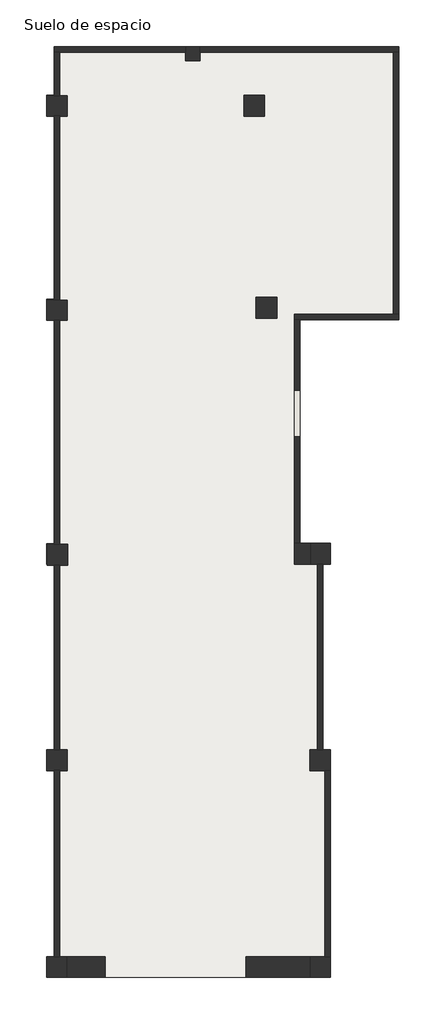
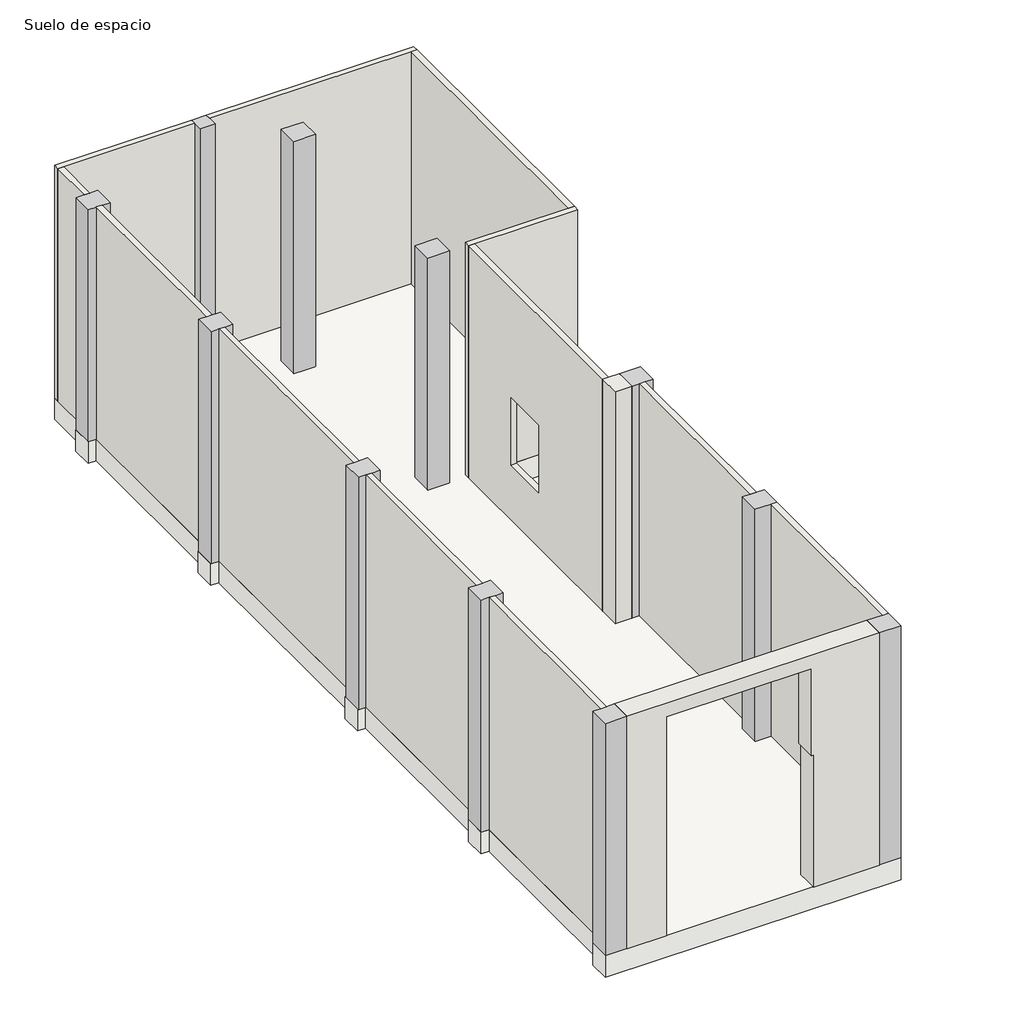
# One storey: 14 walls, 11 columns, 1 slab.
"""IFC4 building model written with IfcOpenShell, lengths in millimetres."""

import ifcopenshell
import ifcopenshell.guid

model = None  # the IFC model being written
_history = None  # IfcOwnerHistory: only IFC2X3 demands one
_inside = {}  # id of a spatial element -> (the spatial element, [elements in it])
_under = {}  # id of a project, library or spatial element -> (it, [spatial elements below it])
_declared = {}  # id of a project -> (the project, [libraries it declares])
_typed = {}  # id of a type object -> (the type object, [elements of that type])
_made_of = {}  # id of a material, layer set ... -> (it, [elements and type objects made of it])


def new_model(schema):
    """Start an empty IFC model of exactly this schema.

    Asked for "IFC4X3", IfcOpenShell would pick the latest addendum, in which some entities
    have other attributes; the version numbers below select the first issue.
    IFC2X3 requires an IfcOwnerHistory on every rooted entity: one is made here for all.
    """
    global model, _history
    if schema == "IFC4X3":
        model = ifcopenshell.file(schema_version=(4, 3, 0, 0))
    else:
        model = ifcopenshell.file(schema=schema)
    _inside.clear()
    _under.clear()
    _declared.clear()
    _typed.clear()
    _made_of.clear()
    _history = None
    if model.schema == "IFC2X3":
        org = make("IfcOrganization", Name="unknown")
        user = make(
            "IfcPersonAndOrganization",
            ThePerson=make("IfcPerson", FamilyName="unknown"),
            TheOrganization=org,
        )
        app = make(
            "IfcApplication",
            ApplicationDeveloper=org,
            Version="unknown",
            ApplicationFullName="unknown",
            ApplicationIdentifier="unknown",
        )
        _history = make(
            "IfcOwnerHistory",
            OwningUser=user,
            OwningApplication=app,
            ChangeAction="ADDED",
            CreationDate=0,
        )
    return model


def make(cls, **values):
    """One entity of the class cls with the attributes given. An attribute that is None is left unset."""
    return model.create_entity(
        cls, **{name: value for name, value in values.items() if value is not None}
    )


def rooted(cls, **values):
    """An entity with a GlobalId (a new one), such as an element, a storey or a relation."""
    return make(cls, GlobalId=ifcopenshell.guid.new(), OwnerHistory=_history, **values)


def si_unit(unit_type, name, prefix=None):
    """IfcSIUnit, for example si_unit("LENGTHUNIT", "METRE", prefix="MILLI")."""
    return make("IfcSIUnit", UnitType=unit_type, Prefix=prefix, Name=name)


def assignment(units):
    """IfcUnitAssignment: the units of a project."""
    return None if units is None else make("IfcUnitAssignment", Units=units)


def point(xyz):
    """IfcCartesianPoint."""
    return None if xyz is None else make("IfcCartesianPoint", Coordinates=xyz)


def direction(xyz):
    """IfcDirection."""
    return None if xyz is None else make("IfcDirection", DirectionRatios=xyz)


def frame(location, z_axis=None, x_axis=None):
    """IfcAxis2Placement3D, a coordinate frame: its origin and axes. An axis left out is left unset."""
    return make(
        "IfcAxis2Placement3D",
        Location=point(location),
        Axis=direction(z_axis),
        RefDirection=direction(x_axis),
    )


def origin():
    """The frame at (0, 0, 0) with its axes left unset."""
    return frame((0.0, 0.0, 0.0))


def origin_with_axes():
    """The frame at (0, 0, 0) with the z axis (0, 0, 1) and the x axis (1, 0, 0) written out."""
    return frame((0.0, 0.0, 0.0), z_axis=(0.0, 0.0, 1.0), x_axis=(1.0, 0.0, 0.0))


def place(relative_to, where):
    """IfcLocalPlacement: puts the frame where relative to a parent placement (None: the world)."""
    return make(
        "IfcLocalPlacement", PlacementRelTo=relative_to, RelativePlacement=where
    )


def context(
    kind, dimensions, precision=None, world=None, true_north=None, identifier=None
):
    """IfcGeometricRepresentationContext, for example the 3D "Model" context."""
    return make(
        "IfcGeometricRepresentationContext",
        ContextIdentifier=identifier,
        ContextType=kind,
        CoordinateSpaceDimension=dimensions,
        Precision=precision,
        WorldCoordinateSystem=world,
        TrueNorth=true_north,
    )


def project(units=None, contexts=None):
    """IfcProject with its units and contexts."""
    return rooted(
        "IfcProject",
        Name="project",
        RepresentationContexts=contexts,
        UnitsInContext=assignment(units),
    )


def spatial(cls, under=None, at=None, **own):
    """A site, building, storey or space (cls), placed at a placement, below another one or the project."""
    s = rooted(cls, ObjectPlacement=at, **own)
    if under is not None:
        _under.setdefault(under.id(), (under, []))[1].append(s)
    return s


def polyline(points):
    """IfcPolyline through the points."""
    return make("IfcPolyline", Points=[point(p) for p in points])


def outline(outer, holes=None, kind="AREA"):
    """IfcArbitraryClosedProfileDef: a profile drawn as a closed curve; with holes, ...WithVoids."""
    if holes is None:
        return make("IfcArbitraryClosedProfileDef", ProfileType=kind, OuterCurve=outer)
    return make(
        "IfcArbitraryProfileDefWithVoids",
        ProfileType=kind,
        OuterCurve=outer,
        InnerCurves=holes,
    )


def extrude(swept, where, along, depth):
    """IfcExtrudedAreaSolid: the profile swept, set in the frame where, extruded along a direction by depth."""
    return make(
        "IfcExtrudedAreaSolid",
        SweptArea=swept,
        Position=where,
        ExtrudedDirection=direction(along),
        Depth=depth,
    )


def faces_of(points, faces, orient=None, outer=None):
    """IfcFace entities. A face is a list of loops; a loop is a list of indices into points, from 0.

    orient and outer hold one flag for each loop. By default every Orientation is true, the
    first loop of a face is its IfcFaceOuterBound and the others are IfcFaceBound.
    """
    made = []
    for i, loops in enumerate(faces):
        bounds = []
        for j, loop in enumerate(loops):
            is_outer = j == 0 if outer is None else outer[i][j]
            bounds.append(
                make(
                    "IfcFaceOuterBound" if is_outer else "IfcFaceBound",
                    Bound=make("IfcPolyLoop", Polygon=[points[k] for k in loop]),
                    Orientation=True if orient is None else orient[i][j],
                )
            )
        made.append(make("IfcFace", Bounds=bounds))
    return made


def faceted_brep(points, faces, orient=None, outer=None, voids=None):
    """IfcFacetedBrep: a solid bounded by flat faces; with voids (closed shells), ...WithVoids."""
    shared = [point(p) for p in points]
    hull = make("IfcClosedShell", CfsFaces=faces_of(shared, faces, orient, outer))
    if voids is None:
        return make("IfcFacetedBrep", Outer=hull)
    return make(
        "IfcFacetedBrepWithVoids",
        Outer=hull,
        Voids=[
            make(cls, CfsFaces=faces_of(shared, fs, o, b)) for cls, fs, o, b in voids
        ],
    )


def shape(context_of_items, identifier, shape_type, items):
    """IfcShapeRepresentation: the items that make up one representation, for example the "Body"."""
    return make(
        "IfcShapeRepresentation",
        ContextOfItems=context_of_items,
        RepresentationIdentifier=identifier,
        RepresentationType=shape_type,
        Items=items,
    )


def source(mapping_origin, context_of_items, identifier, shape_type, items):
    """IfcRepresentationMap: a shape defined once, which mapped items show again and again."""
    return make(
        "IfcRepresentationMap",
        MappingOrigin=mapping_origin,
        MappedRepresentation=shape(context_of_items, identifier, shape_type, items),
    )


def transform(
    local_origin,
    x_axis=None,
    y_axis=None,
    z_axis=None,
    scale=None,
    scale2=None,
    scale3=None,
    uniform=True,
):
    """IfcCartesianTransformationOperator3D, or its non-uniform kind. x_axis, y_axis, z_axis: its Axis1, 2, 3."""
    if uniform:
        return make(
            "IfcCartesianTransformationOperator3D",
            Axis1=direction(x_axis),
            Axis2=direction(y_axis),
            LocalOrigin=point(local_origin),
            Scale=scale,
            Axis3=direction(z_axis),
        )
    return make(
        "IfcCartesianTransformationOperator3DnonUniform",
        Axis1=direction(x_axis),
        Axis2=direction(y_axis),
        LocalOrigin=point(local_origin),
        Scale=scale,
        Axis3=direction(z_axis),
        Scale2=scale2,
        Scale3=scale3,
    )


def mapped(mapping_source, mapping_target):
    """IfcMappedItem: shows the shape of a source again, moved by a transform."""
    return make(
        "IfcMappedItem", MappingSource=mapping_source, MappingTarget=mapping_target
    )


def made_of(thing, what):
    """Note that an element or type object is made of a material, layer set ...; save() writes the relation."""
    if what is not None:
        _made_of.setdefault(what.id(), (what, []))[1].append(thing)
    return thing


def element(
    cls,
    number,
    at=None,
    inside=None,
    cuts=None,
    type_object=None,
    material=None,
    context=None,
    identifier="Body",
    shape_type=None,
    held_by="IfcProductDefinitionShape",
    body=None,
    shapes=None,
    **own,
):
    """One element of the class cls, such as IfcWall. Its Tag is "e" and its number.

    at: its placement. inside: the storey or other place that contains it. cuts: it is an
    opening in that element (IfcRelVoidsElement). A single representation is given by context,
    identifier, shape_type and body (its items); several are given by shapes. held_by: the class
    of the entity that holds the representations. save() writes the other relations.
    """
    e = rooted(cls, Tag="e%d" % number, ObjectPlacement=at, **own)
    if body is not None:
        shapes = [shape(context, identifier, shape_type, body)]
    if shapes is not None:
        e.Representation = make(held_by, Representations=shapes)
    if inside is not None:
        _inside.setdefault(inside.id(), (inside, []))[1].append(e)
    if cuts is not None:
        rooted(
            "IfcRelVoidsElement", RelatingBuildingElement=cuts, RelatedOpeningElement=e
        )
    if type_object is not None:
        _typed.setdefault(type_object.id(), (type_object, []))[1].append(e)
    return made_of(e, material)


def aggregate(whole, parts):
    """IfcRelAggregates: a whole, such as a stair, and the parts it consists of."""
    return rooted("IfcRelAggregates", RelatingObject=whole, RelatedObjects=parts)


def save(model, path):
    """Write the relations noted so far, then the file.

    IfcRelAggregates (storeys below a building ...), IfcRelContainedInSpatialStructure (elements
    in a storey), IfcRelDefinesByType, IfcRelAssociatesMaterial and IfcRelDeclares: one each for
    every whole, place, type object, material and project.
    """
    for whole, parts in _under.values():
        aggregate(whole, parts)
    for where, things in _inside.values():
        rooted(
            "IfcRelContainedInSpatialStructure",
            RelatedElements=things,
            RelatingStructure=where,
        )
    for kind, things in _typed.values():
        rooted("IfcRelDefinesByType", RelatedObjects=things, RelatingType=kind)
    for what, things in _made_of.values():
        rooted("IfcRelAssociatesMaterial", RelatedObjects=things, RelatingMaterial=what)
    for by, libraries in _declared.values():
        rooted("IfcRelDeclares", RelatingContext=by, RelatedDefinitions=libraries)
    model.write(path)


def m_rectangular_column_380_x_380mm_96b74405(model_context):
    return source(origin(), model_context, "Body", "SweptSolid", [
        extrude(outline(polyline([(190.0, 190.0), (190.0, -190.0), (-190.0, -190.0), (-190.0, 190.0), (190.0, 190.0)])), origin_with_axes(), (0.0, 0.0, 1.0), 4300.0),
    ])


model = new_model("IFC4")

# Units and contexts
model_context = context("Model", 3, world=origin())
ifc_project = project(units=[si_unit("LENGTHUNIT", "METRE", prefix="MILLI")], contexts=[model_context])

# Site, building, storey
site = spatial("IfcSite", under=ifc_project)
building = spatial("IfcBuilding", under=site)
storey = spatial("IfcBuildingStorey", under=building, Name="Suelo de espacio", Elevation=0.0)

# Columns
placement = place(None, origin())
element("IfcColumn", 1, ObjectType="M_Rectangular Column : 260 x 260mm", at=placement, inside=storey, context=model_context, shape_type="Brep", body=[
    faceted_brep([(8142.3508412, 14950.939444, 4300.0), (7882.3508412, 14950.939444, 4300.0), (7882.3508412, 14850.939444, 4300.0), (7882.3508412, 14690.939444, 4300.0), (8142.3508412, 14690.939444, 4300.0), (8142.3508412, 14850.939444, 4300.0), (8142.3508412, 14950.939444, 0.0), (8142.3508412, 14850.939444, 0.0), (8142.3508412, 14690.939444, 0.0), (7882.3508412, 14690.939444, 0.0), (7882.3508412, 14850.939444, 0.0), (7882.3508412, 14950.939444, 0.0)], [[[0, 1, 2, 3, 4, 5]], [[6, 7, 8, 9, 10, 11]], [[1, 0, 6, 11]], [[3, 2, 1, 11, 10, 9]], [[4, 3, 9, 8]], [[0, 5, 4, 8, 7, 6]]]),
])
element("IfcColumn", 2, ObjectType="M_Rectangular Column : 380 x 370mm", at=placement, inside=storey, context=model_context, shape_type="Brep", body=[
    faceted_brep([(5722.3508412, 10330.939444, 4300.0), (5342.3508412, 10330.939444, 4300.0), (5342.3508412, 9960.939444, 4300.0), (5482.3508412, 9960.939444, 4300.0), (5582.3508412, 9960.939444, 4300.0), (5722.3508412, 9960.939444, 4300.0), (5722.3508412, 10330.939444, 0.0), (5722.3508412, 9960.939444, 0.0), (5582.3508412, 9960.939444, 0.0), (5482.3508412, 9960.939444, 0.0), (5342.3508412, 9960.939444, 0.0), (5342.3508412, 10330.939444, 0.0)], [[[0, 1, 2, 3, 4, 5]], [[6, 7, 8, 9, 10, 11]], [[1, 0, 6, 11]], [[2, 1, 11, 10]], [[5, 4, 3, 2, 10, 9, 8, 7]], [[0, 5, 7, 6]]]),
])
element("IfcColumn", 3, ObjectType="M_Rectangular Column : 380 x 370mm", at=placement, inside=storey, context=model_context, shape_type="Brep", body=[
    faceted_brep([(5722.3508412, 14050.939444, 4300.0), (5582.3508412, 14050.939444, 4300.0), (5482.3508412, 14050.939444, 4300.0), (5342.3508412, 14050.939444, 4300.0), (5342.3508412, 13680.939444, 4300.0), (5482.3508412, 13680.939444, 4300.0), (5482.3508412, 13685.939444, 4300.0), (5582.3508412, 13685.939444, 4300.0), (5582.3508412, 13680.939444, 4300.0), (5722.3508412, 13680.939444, 4300.0), (5722.3508412, 14050.939444, 0.0), (5722.3508412, 13680.939444, 0.0), (5582.3508412, 13680.939444, 0.0), (5582.3508412, 13685.939444, 0.0), (5482.3508412, 13685.939444, 0.0), (5482.3508412, 13680.939444, 0.0), (5342.3508412, 13680.939444, 0.0), (5342.3508412, 14050.939444, 0.0), (5482.3508412, 14050.939444, 0.0), (5582.3508412, 14050.939444, 0.0)], [[[0, 1, 2, 3, 4, 5, 6, 7, 8, 9]], [[10, 11, 12, 13, 14, 15, 16, 17, 18, 19]], [[3, 2, 1, 0, 10, 19, 18, 17]], [[4, 3, 17, 16]], [[4, 16, 15, 5]], [[0, 9, 11, 10]], [[7, 13, 12, 8]], [[14, 6, 5, 15]], [[13, 7, 6, 14]], [[11, 9, 8, 12]]]),
])
element("IfcColumn", 4, ObjectType="M_Rectangular Column : 380 x 380mm", at=placement, inside=storey, context=model_context, shape_type="Brep", body=[
    faceted_brep([(5722.3508412, -1629.060556, 4300.0), (5582.3508412, -1629.060556, 4300.0), (5482.3508412, -1629.060556, 4300.0), (5342.3508412, -1629.060556, 4300.0), (5342.3508412, -2009.060556, 4300.0), (5722.3508412, -2009.060556, 4300.0), (5722.3508412, -1629.060556, 0.0), (5722.3508412, -2009.060556, 0.0), (5342.3508412, -2009.060556, 0.0), (5342.3508412, -1629.060556, 0.0), (5482.3508412, -1629.060556, 0.0), (5582.3508412, -1629.060556, 0.0)], [[[0, 1, 2, 3, 4, 5]], [[6, 7, 8, 9, 10, 11]], [[3, 2, 1, 0, 6, 11, 10, 9]], [[4, 3, 9, 8]], [[5, 4, 8, 7]], [[0, 5, 7, 6]]]),
])
element("IfcColumn", 5, ObjectType="M_Rectangular Column : 380 x 380mm", at=placement, inside=storey, context=model_context, shape_type="Brep", body=[
    faceted_brep([(10522.3508412, -1629.060556, 4300.0), (10422.3508412, -1629.060556, 4300.0), (10142.3508412, -1629.060556, 4300.0), (10142.3508412, -2009.060556, 4300.0), (10522.3508412, -2009.060556, 4300.0), (10522.3508412, -1629.060556, 0.0), (10522.3508412, -2009.060556, 0.0), (10142.3508412, -2009.060556, 0.0), (10142.3508412, -1629.060556, 0.0), (10422.3508412, -1629.060556, 0.0)], [[[0, 1, 2, 3, 4]], [[5, 6, 7, 8, 9]], [[2, 1, 0, 5, 9, 8]], [[3, 2, 8, 7]], [[4, 3, 7, 6]], [[0, 4, 6, 5]]]),
])
element("IfcColumn", 6, ObjectType="M_Rectangular Column : 380 x 380mm", at=placement, inside=storey, context=model_context, shape_type="Brep", body=[
    faceted_brep([(5722.3508412, 2140.939444, 4300.0), (5582.3508412, 2140.939444, 4300.0), (5482.3508412, 2140.939444, 4300.0), (5342.3508412, 2140.939444, 4300.0), (5342.3508412, 1760.939444, 4300.0), (5482.3508412, 1760.939444, 4300.0), (5482.3508412, 1761.3849652, 4300.0), (5582.3508412, 1761.3849652, 4300.0), (5582.3508412, 1760.939444, 4300.0), (5722.3508412, 1760.939444, 4300.0), (5722.3508412, 2140.939444, 0.0), (5722.3508412, 1760.939444, 0.0), (5582.3508412, 1760.939444, 0.0), (5582.3508412, 1761.3849652, 0.0), (5482.3508412, 1761.3849652, 0.0), (5482.3508412, 1760.939444, 0.0), (5342.3508412, 1760.939444, 0.0), (5342.3508412, 2140.939444, 0.0), (5482.3508412, 2140.939444, 0.0), (5582.3508412, 2140.939444, 0.0)], [[[0, 1, 2, 3, 4, 5, 6, 7, 8, 9]], [[10, 11, 12, 13, 14, 15, 16, 17, 18, 19]], [[3, 2, 1, 0, 10, 19, 18, 17]], [[4, 3, 17, 16]], [[4, 16, 15, 5]], [[0, 9, 11, 10]], [[7, 13, 12, 8]], [[14, 6, 5, 15]], [[11, 9, 8, 12]], [[13, 7, 6, 14]]]),
])
element("IfcColumn", 7, ObjectType="M_Rectangular Column : 380 x 380mm", at=placement, inside=storey, context=model_context, shape_type="Brep", body=[
    faceted_brep([(10522.3508412, 2140.939444, 4300.0), (10382.3508412, 2140.939444, 4300.0), (10282.3508412, 2140.939444, 4300.0), (10142.3508412, 2140.939444, 4300.0), (10142.3508412, 1760.939444, 4300.0), (10422.3508412, 1760.939444, 4300.0), (10522.3508412, 1760.939444, 4300.0), (10522.3508412, 2140.939444, 0.0), (10522.3508412, 1760.939444, 0.0), (10422.3508412, 1760.939444, 0.0), (10142.3508412, 1760.939444, 0.0), (10142.3508412, 2140.939444, 0.0), (10282.3508412, 2140.939444, 0.0), (10382.3508412, 2140.939444, 0.0)], [[[0, 1, 2, 3, 4, 5, 6]], [[7, 8, 9, 10, 11, 12, 13]], [[3, 2, 1, 0, 7, 13, 12, 11]], [[4, 3, 11, 10]], [[6, 5, 4, 10, 9, 8]], [[0, 6, 8, 7]]]),
])
element("IfcColumn", 8, ObjectType="M_Rectangular Column : 380 x 380mm", at=placement, inside=storey, context=model_context, shape_type="Brep", body=[
    faceted_brep([(5732.3508412, 5880.939444, 4300.0), (5582.3508412, 5880.939444, 4300.0), (5482.3508412, 5880.939444, 4300.0), (5352.3508412, 5880.939444, 4300.0), (5352.3508412, 5500.939444, 4300.0), (5482.3508412, 5500.939444, 4300.0), (5582.3508412, 5500.939444, 4300.0), (5732.3508412, 5500.939444, 4300.0), (5732.3508412, 5880.939444, 0.0), (5732.3508412, 5500.939444, 0.0), (5582.3508412, 5500.939444, 0.0), (5482.3508412, 5500.939444, 0.0), (5352.3508412, 5500.939444, 0.0), (5352.3508412, 5880.939444, 0.0), (5482.3508412, 5880.939444, 0.0), (5582.3508412, 5880.939444, 0.0)], [[[0, 1, 2, 3, 4, 5, 6, 7]], [[8, 9, 10, 11, 12, 13, 14, 15]], [[3, 2, 1, 0, 8, 15, 14, 13]], [[4, 3, 13, 12]], [[7, 6, 5, 4, 12, 11, 10, 9]], [[0, 7, 9, 8]]]),
])
element("IfcColumn", 9, ObjectType="M_Rectangular Column : 380 x 380mm", at=placement, inside=storey, context=model_context, shape_type="Brep", body=[
    faceted_brep([(10522.3508412, 5520.939444, 4300.0), (10522.3508412, 5900.939444, 4300.0), (10152.3508412, 5900.939444, 4300.0), (10152.3508412, 5520.939444, 4300.0), (10282.3508412, 5520.939444, 4300.0), (10382.3508412, 5520.939444, 4300.0), (10522.3508412, 5900.939444, 0.0), (10522.3508412, 5520.939444, 0.0), (10382.3508412, 5520.939444, 0.0), (10282.3508412, 5520.939444, 0.0), (10152.3508412, 5520.939444, 0.0), (10152.3508412, 5900.939444, 0.0)], [[[0, 1, 2, 3, 4, 5]], [[6, 7, 8, 9, 10, 11]], [[1, 6, 11, 2]], [[7, 0, 5, 4, 3, 10, 9, 8]], [[1, 0, 7, 6]], [[3, 2, 11, 10]]]),
])
m_rectangular_column_380_x_380mm_shape = m_rectangular_column_380_x_380mm_96b74405(model_context)
element("IfcColumn", 10, ObjectType="M_Rectangular Column : 380 x 380mm", at=placement, inside=storey, context=model_context, shape_type="MappedRepresentation", body=[
    mapped(m_rectangular_column_380_x_380mm_shape, transform((9132.3508412, 13870.939444, 0.0), x_axis=(1.0, 0.0, 0.0), y_axis=(0.0, 1.0, 0.0), z_axis=(0.0, 0.0, 1.0))),
])
element("IfcColumn", 11, ObjectType="M_Rectangular Column : 380 x 380mm", at=placement, inside=storey, context=model_context, shape_type="MappedRepresentation", body=[
    mapped(m_rectangular_column_380_x_380mm_shape, transform((9352.3508412, 10190.939444, 0.0), x_axis=(1.0, 0.0, 0.0), y_axis=(0.0, 1.0, 0.0), z_axis=(0.0, 0.0, 1.0))),
])

# Slab
element("IfcSlab", 12, ObjectType="Generic Floor - 400mm", at=placement, inside=storey, context=model_context, shape_type="SweptSolid", body=[
    extrude(outline(polyline([(11772.3508412, 14950.939444), (11772.3508412, 9970.939444), (9962.3508412, 9970.939444), (9962.3508412, 5900.939444), (10382.3508412, 5900.939444), (10382.3508412, 2140.939444), (10522.3508412, 2140.939444), (10522.3508412, -2009.060556), (5342.3508412, -2009.060556), (5342.3508412, -1629.060556), (5482.3508412, -1629.060556), (5482.3508412, 1761.3849652), (5342.3508412, 1761.3849652), (5342.3508412, 2140.939444), (5482.3508412, 2140.939444), (5482.3508412, 5516.6200626), (5342.3508412, 5516.6200626), (5342.3508412, 5896.6200626), (5482.3508412, 5896.6200626), (5482.3508412, 9965.939444), (5342.3508412, 9965.939444), (5342.3508412, 10345.939444), (5482.3508412, 10345.939444), (5482.3508412, 13690.939444), (5342.3508412, 13690.939444), (5342.3508412, 14060.939444), (5482.3508412, 14060.939444), (5482.3508412, 14950.939444), (11772.3508412, 14950.939444)])), frame((0.0, 0.0, -400.0), z_axis=(0.0, 0.0, 1.0), x_axis=(1.0, 0.0, 0.0)), (0.0, 0.0, 1.0), 400.0),
])

# Walls
element("IfcWall", 13, ObjectType="Generic - 100mm Masonry", at=placement, inside=storey, context=model_context, shape_type="Brep", body=[
    faceted_brep([(5582.3508412, -1629.060556, 0.0), (5582.3508412, 1760.939444, 0.0), (5582.3508412, 1761.3849652, 0.0), (5582.3508412, 1761.3849652, 4300.0), (5582.3508412, 1760.939444, 4300.0), (5582.3508412, -1629.060556, 4300.0), (5482.3508412, -1629.060556, 0.0), (5482.3508412, -1629.060556, 4300.0), (5482.3508412, 1760.939444, 4300.0), (5482.3508412, 1761.3849652, 4300.0), (5482.3508412, 1761.3849652, 0.0), (5482.3508412, 1760.939444, 0.0)], [[[0, 1, 2, 3, 4, 5]], [[6, 7, 8, 9, 10, 11]], [[2, 1, 0, 6, 11, 10]], [[3, 2, 10, 9]], [[5, 4, 3, 9, 8, 7]], [[0, 5, 7, 6]]]),
])
element("IfcWall", 14, ObjectType="Generic - 100mm Masonry", at=placement, inside=storey, context=model_context, shape_type="SweptSolid", body=[
    extrude(outline(polyline([(5582.3508412, 5500.939444), (5582.3508412, 2140.939444), (5482.3508412, 2140.939444), (5482.3508412, 5500.939444), (5582.3508412, 5500.939444)])), origin_with_axes(), (0.0, 0.0, 1.0), 4300.0),
])
element("IfcWall", 15, ObjectType="Generic - 100mm Masonry", at=placement, inside=storey, context=model_context, shape_type="SweptSolid", body=[
    extrude(outline(polyline([(5582.3508412, 9960.939444), (5582.3508412, 5880.939444), (5482.3508412, 5880.939444), (5482.3508412, 9960.939444), (5582.3508412, 9960.939444)])), origin_with_axes(), (0.0, 0.0, 1.0), 4300.0),
])
element("IfcWall", 16, ObjectType="Generic - 100mm Masonry", at=placement, inside=storey, context=model_context, shape_type="Brep", body=[
    faceted_brep([(5582.3508412, 10335.939444, 0.0), (5582.3508412, 13680.939444, 0.0), (5582.3508412, 13685.939444, 0.0), (5582.3508412, 13685.939444, 4300.0), (5582.3508412, 13680.939444, 4300.0), (5582.3508412, 10335.939444, 4300.0), (5482.3508412, 10335.939444, 0.0), (5482.3508412, 10335.939444, 4300.0), (5482.3508412, 13680.939444, 4300.0), (5482.3508412, 13685.939444, 4300.0), (5482.3508412, 13685.939444, 0.0), (5482.3508412, 13680.939444, 0.0)], [[[0, 1, 2, 3, 4, 5]], [[6, 7, 8, 9, 10, 11]], [[2, 1, 0, 6, 11, 10]], [[3, 2, 10, 9]], [[5, 4, 3, 9, 8, 7]], [[0, 5, 7, 6]]]),
])
element("IfcWall", 17, ObjectType="Generic - 100mm Masonry", at=placement, inside=storey, context=model_context, shape_type="SweptSolid", body=[
    extrude(outline(polyline([(5582.3508412, 14850.939444), (5582.3508412, 14050.939444), (5482.3508412, 14050.939444), (5482.3508412, 14850.939444), (5582.3508412, 14850.939444)])), origin_with_axes(), (0.0, 0.0, 1.0), 4300.0),
])
element("IfcWall", 18, ObjectType="Generic - 100mm Masonry", at=placement, inside=storey, context=model_context, shape_type="Brep", body=[
    faceted_brep([(5482.3508412, 14850.939444, 0.0), (5582.3508412, 14850.939444, 0.0), (7882.3508412, 14850.939444, 0.0), (7882.3508412, 14850.939444, 4300.0), (5582.3508412, 14850.939444, 4300.0), (5482.3508412, 14850.939444, 4300.0), (5482.3508412, 14950.939444, 0.0), (5482.3508412, 14950.939444, 4300.0), (7882.3508412, 14950.939444, 4300.0), (7882.3508412, 14950.939444, 0.0)], [[[0, 1, 2, 3, 4, 5]], [[6, 7, 8, 9]], [[2, 1, 0, 6, 9]], [[3, 2, 9, 8]], [[5, 4, 3, 8, 7]], [[0, 5, 7, 6]]]),
])
element("IfcWall", 19, ObjectType="Generic - 100mm Masonry", at=placement, inside=storey, context=model_context, shape_type="Brep", body=[
    faceted_brep([(8142.3508412, 14850.939444, 0.0), (11672.3508412, 14850.939444, 0.0), (11772.3508412, 14850.939444, 0.0), (11772.3508412, 14850.939444, 4300.0), (11672.3508412, 14850.939444, 4300.0), (8142.3508412, 14850.939444, 4300.0), (8142.3508412, 14950.939444, 0.0), (8142.3508412, 14950.939444, 4300.0), (11772.3508412, 14950.939444, 4300.0), (11772.3508412, 14950.939444, 0.0)], [[[0, 1, 2, 3, 4, 5]], [[6, 7, 8, 9]], [[2, 1, 0, 6, 9]], [[5, 4, 3, 8, 7]], [[0, 5, 7, 6]], [[3, 2, 9, 8]]]),
])
element("IfcWall", 20, ObjectType="Generic - 100mm Masonry", at=placement, inside=storey, context=model_context, shape_type="SweptSolid", body=[
    extrude(outline(polyline([(11672.3508412, 10070.939444), (11672.3508412, 14850.939444), (11772.3508412, 14850.939444), (11772.3508412, 10070.939444), (11672.3508412, 10070.939444)])), origin_with_axes(), (0.0, 0.0, 1.0), 4300.0),
])
element("IfcWall", 21, ObjectType="Generic - 100mm Masonry", at=placement, inside=storey, context=model_context, shape_type="Brep", body=[
    faceted_brep([(11772.3508412, 10070.939444, 0.0), (11672.3508412, 10070.939444, 0.0), (9862.3508412, 10070.939444, 0.0), (9862.3508412, 10070.939444, 4300.0), (11672.3508412, 10070.939444, 4300.0), (11772.3508412, 10070.939444, 4300.0), (11772.3508412, 9970.939444, 0.0), (11772.3508412, 9970.939444, 4300.0), (9962.3508412, 9970.939444, 4300.0), (9862.3508412, 9970.939444, 4300.0), (9862.3508412, 9970.939444, 0.0), (9962.3508412, 9970.939444, 0.0)], [[[0, 1, 2, 3, 4, 5]], [[6, 7, 8, 9, 10, 11]], [[2, 1, 0, 6, 11, 10]], [[5, 4, 3, 9, 8, 7]], [[3, 2, 10, 9]], [[0, 5, 7, 6]]]),
])
element("IfcWall", 22, ObjectType="Generic - 100mm Masonry", at=placement, inside=storey, context=model_context, shape_type="SweptSolid", body=[
    extrude(outline(polyline([(9970.939444, 0.0), (5900.939444, 0.0), (5900.939444, 4300.0), (9970.939444, 4300.0), (9970.939444, 0.0)]), holes=[polyline([(8685.5060628, 2270.0), (7845.5060628, 2270.0), (7845.5060628, 1020.0), (8685.5060628, 1020.0), (8685.5060628, 2270.0)])]), frame((9862.3508412, 0.0, 0.0), z_axis=(1.0, 0.0, 0.0), x_axis=(0.0, 1.0, 0.0)), (0.0, 0.0, 1.0), 100.0),
])
element("IfcWall", 23, ObjectType="Generic - 100mm Masonry", at=placement, inside=storey, context=model_context, shape_type="SweptSolid", body=[
    extrude(outline(polyline([(10282.3508412, 2140.939444), (10282.3508412, 5520.939444), (10382.3508412, 5520.939444), (10382.3508412, 2140.939444), (10282.3508412, 2140.939444)])), origin_with_axes(), (0.0, 0.0, 1.0), 4300.0),
])
element("IfcWall", 24, ObjectType="Generic - 100mm Masonry", at=placement, inside=storey, context=model_context, shape_type="SweptSolid", body=[
    extrude(outline(polyline([(10422.3508412, -1629.060556), (10422.3508412, 1760.939444), (10522.3508412, 1760.939444), (10522.3508412, -1629.060556), (10422.3508412, -1629.060556)])), origin_with_axes(), (0.0, 0.0, 1.0), 4300.0),
])
element("IfcWall", 25, ObjectType="Generic - 380mm Masonry", at=placement, inside=storey, context=model_context, shape_type="Brep", body=[
    faceted_brep([(9862.3508412, 5520.939444, 0.0), (10152.3508412, 5520.939444, 0.0), (10152.3508412, 5520.939444, 4300.0), (9862.3508412, 5520.939444, 4300.0), (9862.3508412, 5900.939444, 0.0), (9862.3508412, 5900.939444, 4300.0), (9962.3508412, 5900.939444, 4300.0), (10152.3508412, 5900.939444, 4300.0), (10152.3508412, 5900.939444, 0.0), (9962.3508412, 5900.939444, 0.0)], [[[0, 1, 2, 3]], [[4, 5, 6, 7, 8, 9]], [[1, 0, 4, 9, 8]], [[2, 1, 8, 7]], [[3, 2, 7, 6, 5]], [[0, 3, 5, 4]]]),
])
element("IfcWall", 26, ObjectType="Generic - 380mm Masonry", at=placement, inside=storey, context=model_context, shape_type="Brep", body=[
    faceted_brep([(10142.3508412, -2009.060556, 0.0), (10142.3508412, -2009.060556, 4300.0), (5722.3508412, -2009.060556, 4300.0), (5722.3508412, -2009.060556, 0.0), (6412.3508412, -2009.060556, 0.0), (6412.3508412, -2009.060556, 3080.0), (6412.3508412, -2009.060556, 4050.0), (8952.3508412, -2009.060556, 4050.0), (8952.3508412, -2009.060556, 3080.0), (8952.3508412, -2009.060556, 2438.4), (8983.3912604, -2009.060556, 2438.4), (8983.3912604, -2009.060556, 0.0), (10142.3508412, -1629.060556, 4300.0), (10142.3508412, -1629.060556, 0.0), (8983.3912604, -1629.060556, 0.0), (8983.3912604, -1629.060556, 2438.4), (8952.3508412, -1629.060556, 2438.4), (8952.3508412, -1629.060556, 4050.0), (6412.3508412, -1629.060556, 4050.0), (6412.3508412, -1629.060556, 0.0), (5722.3508412, -1629.060556, 0.0), (5722.3508412, -1629.060556, 4300.0), (6412.3508412, -1929.060556, 4050.0), (8952.3508412, -1929.060556, 4050.0)], [[[0, 1, 2, 3, 4, 5, 6, 7, 8, 9, 10, 11]], [[12, 13, 14, 15, 16, 17, 18, 19, 20, 21]], [[3, 20, 19, 4]], [[13, 0, 11, 14]], [[1, 0, 13, 12]], [[2, 1, 12, 21]], [[3, 2, 21, 20]], [[15, 10, 9, 16]], [[10, 15, 14, 11]], [[6, 22, 18, 17, 23, 7]], [[18, 22, 6, 5, 4, 19]], [[7, 23, 17, 16, 9, 8]]]),
])

save(model, "model.ifc")

# Revit data of these elements
# Project information
#   Organization Name = "SHV"
#   Building Name = "Pere Valencia"
#   Author = "Ian Salter"
#   Project Issue Date = "15/07/2022"
#   Project Status = "Project  Status"
#   Client Name = "Ian Salter"
#   Project Address = "## Street\nCity, State  Zip"
#   Project Name = "SHV"
#   Project Number = "1"
# Type "M_Rectangular Column : 260 x 260mm"
#   Depth = 26 cm
#   Offset Base = 0 cm
#   Offset Top = 0 cm
#   Width = 26 cm
#   Material = none
# Type "M_Rectangular Column : 380 x 370mm"
#   Depth = 37 cm
#   Offset Base = 0 cm
#   Offset Top = 0 cm
#   Width = 38 cm
#   Material = none
# Type "M_Rectangular Column : 380 x 380mm"
#   Depth = 38 cm
#   Offset Base = 0 cm
#   Offset Top = 0 cm
#   Width = 38 cm
#   Material = none
# Type "Generic Floor - 400mm"
#   Function = 0
#   Layers, outside or top first: 40 cm no material (function 1)
# Type "Generic - 100mm Masonry"
#   Layers, outside or top first: 10 cm "Concrete, Cast-in-Place gray" (function 1)
# Type "Generic - 380mm Masonry"
#   Layers, outside or top first: 38 cm "Concrete, Cast-in-Place gray" (function 1)
# Element 1 (IfcColumn, "M_Rectangular Column : 260 x 260mm")
#   Phase Created = Existing
#   Materials on its faces: "Concrete, Cast-in-Place gray"
# Element 2 (IfcColumn, "M_Rectangular Column : 380 x 370mm")
#   Phase Created = Existing
#   Materials on its faces: "Default Wall"
# Element 3 (IfcColumn, "M_Rectangular Column : 380 x 370mm")
#   Phase Created = Existing
#   Materials on its faces: "Concrete, Cast-in-Place gray"
# Elements 4, 5 (IfcColumn, "M_Rectangular Column : 380 x 380mm")
#   Phase Created = New Construction
#   Materials on its faces: "Concrete, Cast-in-Place gray"
# Elements 6, 7, 8, 9 (IfcColumn, "M_Rectangular Column : 380 x 380mm")
#   Phase Created = Existing
#   Materials on its faces: "Concrete, Cast-in-Place gray"
# Elements 10, 11 (IfcColumn, "M_Rectangular Column : 380 x 380mm")
#   Phase Created = Existing
# Element 12 (IfcSlab, "Generic Floor - 400mm")
#   Height Offset From Level = 0 cm
#   Phase Created = New Construction
#   Materials on its faces: "Default Roof"
# Elements 13, 14, 15, 16, 17, 18, 19, 20, 21, 22, 23, 24 (IfcWall, "Generic - 100mm Masonry")
#   Top Offset = 0 cm
#   Base Offset = 0 cm
#   wall height = 430 cm
#   Phase Created = Existing
#   Base Constraint = Suelo de espacio
#   Top Constraint = Techo de espacio
#   Materials on its faces: "Concrete, Cast-in-Place gray"
# Element 25 (IfcWall, "Generic - 380mm Masonry")
#   Top Offset = 0 cm
#   Base Offset = 0 cm
#   wall height = 430 cm
#   Phase Created = Existing
#   Base Constraint = Suelo de espacio
#   Top Constraint = Techo de espacio
#   Materials on its faces: "Concrete, Cast-in-Place gray"
# Element 26 (IfcWall, "Generic - 380mm Masonry")
#   Top Offset = 0 cm
#   Base Offset = 0 cm
#   Unconnected Height = 430 cm
#   wall height = 430 cm
#   Phase Created = Existing
#   Base Constraint = Suelo de espacio
#   Materials on its faces: "Concrete, Cast-in-Place gray"
# Materials
#   "Concrete, Cast-in-Place gray": class "Concrete", colour RGB 115 116 108, transparency 0, Description = "Cast-in-place concrete", Cost = 0
#   "Default Wall": class "Miscellaneous", colour RGB 80 80 80, transparency 0
#   "Default Roof": class "Miscellaneous", colour RGB 80 80 80, transparency 0
